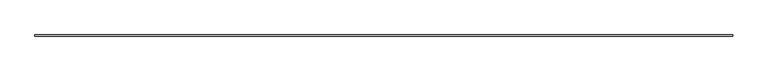
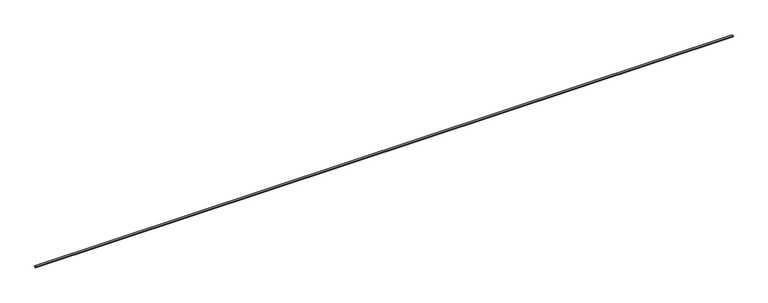
"""IFC4 building model written with IfcOpenShell, lengths in millimetres: proxy geometry, Joint012 33866 : Joint012 33866."""

from ifc_helpers import new_model, si_unit, point, frame, frame_2d, origin, place, context, project, spatial, polyline, circle_curve, trimmed, segment, composite_curve, outline, extrude, source, transform, mapped, element, save


def generic_models_801eaf96(model_context):
    return source(origin(), model_context, "Body", "SweptSolid", [
        extrude(outline(composite_curve([segment(trimmed(circle_curve(frame_2d((-4627.2943844, 38428.99375)), 5.4132205), [point((-4625.6960524, 38423.821875))], [point((-4628.8927164, 38423.821875))], False, "CARTESIAN"), True, "CONTINUOUS"), segment(polyline([(-4628.8927164, 38423.821875), (-4628.8927164, 38427.7398437)]), True, "CONTINUOUS"), segment(trimmed(circle_curve(frame_2d((-4627.2943844, 38432.9117187)), 5.4132205), [point((-4628.8927164, 38427.7398437))], [point((-4625.6960524, 38427.7398437))], True, "CARTESIAN"), True, "CONTINUOUS"), segment(polyline([(-4625.6960524, 38427.7398437), (-4625.6960524, 38423.821875)]), True, "CONTINUOUS")], self_intersect=False)), frame((12383.0178845, 0.0, 0.0), z_axis=(1.0, 0.0, 0.0), x_axis=(0.0, 1.0, 0.0)), (0.0, 0.0, 1.0), 2000.0),
    ])


if __name__ == "__main__":
    model = new_model("IFC4")
    model_context = context("Model", 3, world=origin())
    ifc_project = project(units=[si_unit("LENGTHUNIT", "METRE", prefix="MILLI")], contexts=[model_context])
    site = spatial("IfcSite", under=ifc_project)
    building = spatial("IfcBuilding", under=site)
    placement = place(None, origin())
    generic_models_shape = generic_models_801eaf96(model_context)
    element("IfcBuildingElementProxy", 1, Name="Joint012 33866 : Joint012 33866", ObjectType="Joint012 33866 : Joint012 33866", at=placement, inside=building, context=model_context, shape_type="MappedRepresentation", body=[
        mapped(generic_models_shape, transform((0.0, 0.0, 0.0), x_axis=(1.0, 0.0, 0.0), y_axis=(0.0, 1.0, 0.0), z_axis=(0.0, 0.0, 1.0))),
    ])
    save(model, "model.ifc")

# Revit data of these elements
# Type "Joint012 33866 : Joint012 33866"
#   NameOverride = "Joint012"
# Element 1 (IfcBuildingElementProxy, "Joint012 33866 : Joint012 33866")
#   Materials on its faces: "SEALANT JOINT"
# Materials
#   "SEALANT JOINT": class "Unassigned", colour RGB 142 225 148, transparency 0
